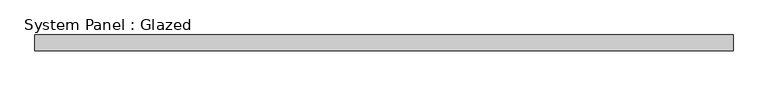
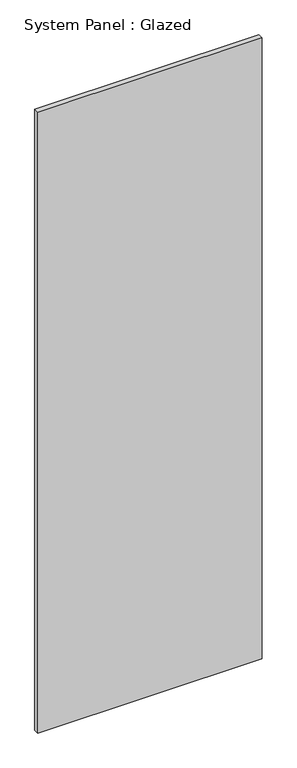
"""IFC4 building model written with IfcOpenShell, lengths in millimetres: plate geometry, System Panel : Glazed."""

from ifc_helpers import new_model, si_unit, origin, origin_with_axes, place, context, project, spatial, polyline, outline, extrude, source, transform, mapped, element, save


def system_panel_glazed_b92d501e(model_context):
    return source(origin(), model_context, "Body", "SweptSolid", [
        extrude(outline(polyline([(567.2666667, 19.05), (-567.2666667, 19.05), (-567.2666667, 44.45), (567.2666667, 44.45), (567.2666667, 19.05)])), origin_with_axes(), (0.0, 0.0, 1.0), 3318.9333333),
    ])


if __name__ == "__main__":
    model = new_model("IFC4")
    model_context = context("Model", 3, world=origin())
    ifc_project = project(units=[si_unit("LENGTHUNIT", "METRE", prefix="MILLI")], contexts=[model_context])
    site = spatial("IfcSite", under=ifc_project)
    building = spatial("IfcBuilding", under=site)
    placement = place(None, origin())
    system_panel_glazed_shape = system_panel_glazed_b92d501e(model_context)
    element("IfcPlate", 1, ObjectType="System Panel : Glazed", at=placement, inside=building, context=model_context, shape_type="MappedRepresentation", body=[
        mapped(system_panel_glazed_shape, transform((0.0, 0.0, 0.0), x_axis=(1.0, 0.0, 0.0), y_axis=(0.0, 1.0, 0.0), z_axis=(0.0, 0.0, 1.0))),
    ])
    save(model, "model.ifc")

# Revit data of these elements
# Type "System Panel : Glazed"
#   Construction Type Id = "GSP4R"
#   Analytic Construction = "1/8 in Pilkington single glazing"
#   Visual Light Transmittance = 0.9
#   Solar Heat Gain Coefficient = 0.86
#   Heat Transfer Coefficient (U) = 1.18115 BTU/(h·ft²·°F)
#   Define Thermal Properties by = 1
# Element 1 (IfcPlate, "System Panel : Glazed")
#   Materials on its faces: "Glass"
# Materials
#   "Glass": class "Glass", colour RGB 0 128 192, transparency 0.75, Description = "Soda Lime Glass", Cost = 0
